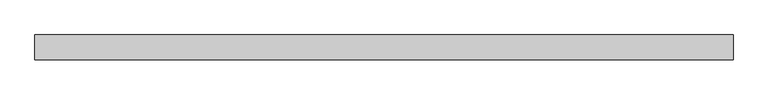
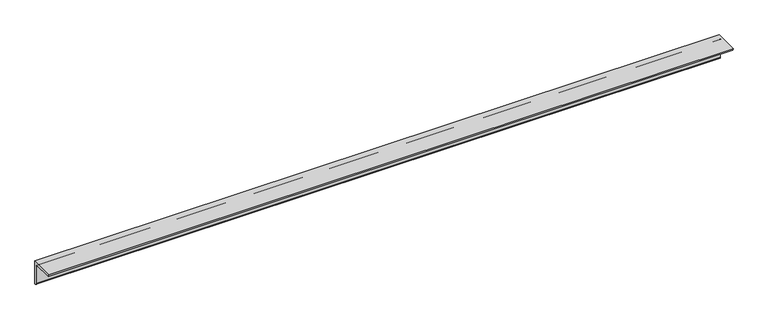
"""IFC4 building model written with IfcOpenShell, lengths in millimetres: member geometry, 0912_Steel Framing_L-KSD3502 : H_SB_AR_S03_L-130x130x12_HBR3."""

from ifc_helpers import new_model, si_unit, point, frame, frame_2d, origin, place, context, project, spatial, polyline, circle_curve, trimmed, segment, composite_curve, outline, extrude, source, transform, mapped, element, save


def member_c24f28f7(model_context):
    return source(origin(), model_context, "Body", "SweptSolid", [
        extrude(outline(composite_curve([segment(polyline([(36.4, 36.4), (36.4, -93.6)]), True, "CONTINUOUS"), segment(trimmed(circle_curve(frame_2d((36.4, -81.6)), 12.0), [point((36.4, -93.6))], [point((24.4, -81.6))], False, "CARTESIAN"), True, "CONTINUOUS"), segment(polyline([(24.4, -81.6), (24.4, 12.4)]), True, "CONTINUOUS"), segment(trimmed(circle_curve(frame_2d((12.4, 12.4)), 12.0), [point((24.4, 12.4))], [point((12.4, 24.4))], True, "CARTESIAN"), True, "CONTINUOUS"), segment(polyline([(12.4, 24.4), (-81.6, 24.4)]), True, "CONTINUOUS"), segment(trimmed(circle_curve(frame_2d((-81.6, 36.4)), 12.0), [point((-81.6, 24.4))], [point((-93.6, 36.4))], False, "CARTESIAN"), True, "CONTINUOUS"), segment(polyline([(-93.6, 36.4), (36.4, 36.4)]), True, "CONTINUOUS")], self_intersect=False)), frame((-1867.6865023, 0.0, 0.0), z_axis=(1.0, 0.0, 0.0), x_axis=(0.0, 1.0, 0.0)), (0.0, 0.0, 1.0), 3659.8690046),
    ])


if __name__ == "__main__":
    model = new_model("IFC4")
    model_context = context("Model", 3, world=origin())
    ifc_project = project(units=[si_unit("LENGTHUNIT", "METRE", prefix="MILLI")], contexts=[model_context])
    site = spatial("IfcSite", under=ifc_project)
    building = spatial("IfcBuilding", under=site)
    placement = place(None, origin())
    member_shape = member_c24f28f7(model_context)
    element("IfcMember", 1, ObjectType="0912_Steel Framing_L-KSD3502 : H_SB_AR_S03_L-130x130x12_HBR3", at=placement, inside=building, context=model_context, shape_type="MappedRepresentation", body=[
        mapped(member_shape, transform((0.0, 0.0, 0.0), x_axis=(1.0, 0.0, 0.0), y_axis=(0.0, 1.0, 0.0), z_axis=(0.0, 0.0, 1.0))),
    ])
    save(model, "model.ifc")

# Revit data of these elements
# Type "0912_Steel Framing_L-KSD3502 : H_SB_AR_S03_L-130x130x12_HBR3"
#   k = 25 mm
#   Perimeter = 0.52 m²/m
#   Nominal Weight = 23.40 kgf/m
#   Length [instance default] = 1000 mm
#   b = 130 mm
#   d = 130 mm
#   t = 12 mm
#   x = 36.4 mm
#   y = 36.4 mm
#   A = 2976.00 m²
#   Structural Material [instance default] = Steel, 45-345
# Element 1 (IfcMember, "0912_Steel Framing_L-KSD3502 : H_SB_AR_S03_L-130x130x12_HBR3")
#   Structural Material = Steel ASTM A36
#   Materials on its faces: "Steel ASTM A36"
# Materials
#   "Steel, 45-345": class "Metal", colour RGB 189 187 185, transparency 0, Description = "Steel 345 MPa", Cost = 0
#   "Steel ASTM A36": class "Metal", colour RGB 199 199 199, transparency 0, Description = "Structural steel, ASTM A36 Grade B, mill finish", Cost = 0
